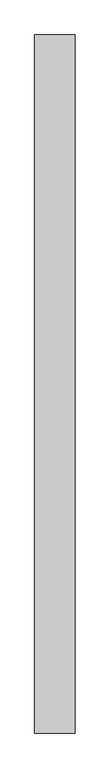
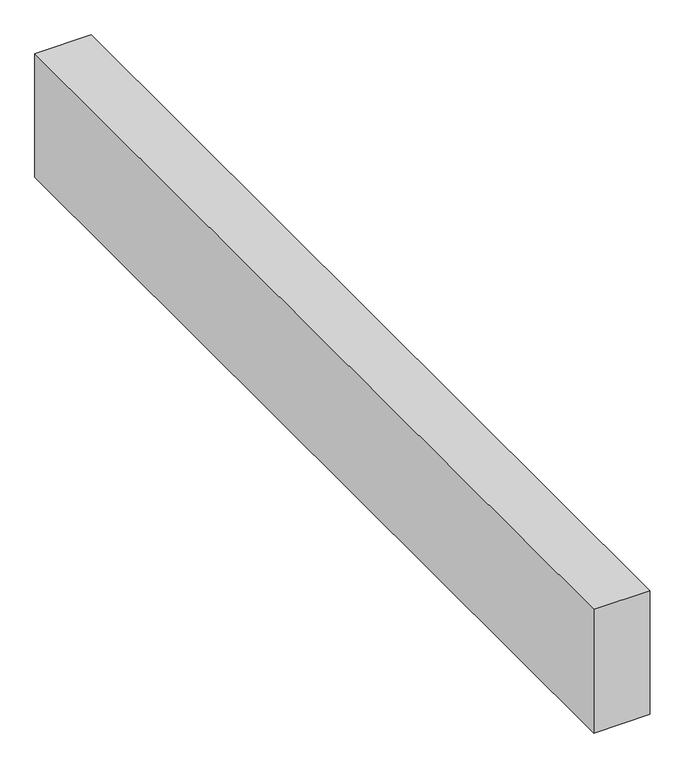
"""IFC4 building model written with IfcOpenShell, lengths in millimetres: proxy geometry, Structure003 1066 : Structure003 1066."""

from ifc_helpers import new_model, si_unit, frame, origin, place, context, project, spatial, polyline, outline, extrude, source, transform, mapped, element, save


def generic_models_f1f9d59e(model_context):
    return source(origin(), model_context, "Body", "SweptSolid", [
        extrude(outline(polyline([(4322.6883192, 7656.2019481), (4322.6883192, 10284.3743438), (4475.0883192, 10284.3743438), (4475.0883192, 7656.2019481), (4322.6883192, 7656.2019481)])), frame((0.0, 0.0, 39757.096), z_axis=(0.0, 0.0, 1.0), x_axis=(1.0, 0.0, 0.0)), (0.0, 0.0, 1.0), 355.6),
    ])


if __name__ == "__main__":
    model = new_model("IFC4")
    model_context = context("Model", 3, world=origin())
    ifc_project = project(units=[si_unit("LENGTHUNIT", "METRE", prefix="MILLI")], contexts=[model_context])
    site = spatial("IfcSite", under=ifc_project)
    building = spatial("IfcBuilding", under=site)
    placement = place(None, origin())
    generic_models_shape = generic_models_f1f9d59e(model_context)
    element("IfcBuildingElementProxy", 1, Name="Structure003 1066 : Structure003 1066", ObjectType="Structure003 1066 : Structure003 1066", at=placement, inside=building, context=model_context, shape_type="MappedRepresentation", body=[
        mapped(generic_models_shape, transform((0.0, 0.0, 0.0), x_axis=(1.0, 0.0, 0.0), y_axis=(0.0, 1.0, 0.0), z_axis=(0.0, 0.0, 1.0))),
    ])
    save(model, "model.ifc")

# Revit data of these elements
# Type "Structure003 1066 : Structure003 1066"
#   NameOverride = "Structure003"
# Element 1 (IfcBuildingElementProxy, "Structure003 1066 : Structure003 1066")
#   Materials on its faces: "STRUCTURAL MEMBER (SEE DWGS)"
# Materials
#   "STRUCTURAL MEMBER (SEE DWGS)": class "Unassigned", colour RGB 214 178 158, transparency 0, Cost = 0
